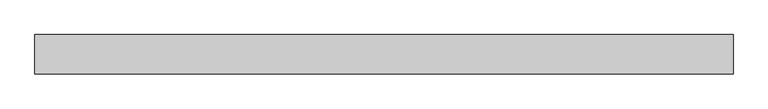
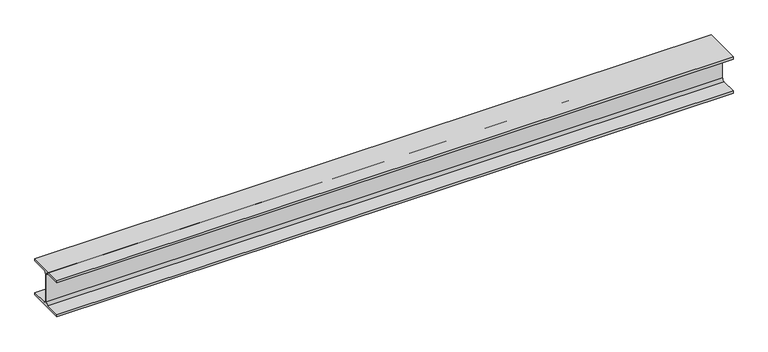
"""IFC4 building model written with IfcOpenShell, lengths in millimetres: beam geometry, 0912_Steel Framing_H-KSD3502 : H_SB_ASB_H-200x200x8x12."""

from ifc_helpers import new_model, si_unit, point, frame, frame_2d, origin, place, context, project, spatial, polyline, circle_curve, trimmed, segment, composite_curve, outline, extrude, source, transform, mapped, element, save


def beam_e80e70f2(model_context):
    return source(origin(), model_context, "Body", "SweptSolid", [
        extrude(outline(composite_curve([segment(polyline([(100.0, -88.0), (100.0, -100.0), (-100.0, -100.0), (-100.0, -88.0), (-17.0, -88.0)]), True, "CONTINUOUS"), segment(trimmed(circle_curve(frame_2d((-17.0, -75.0)), 13.0), [point((-17.0, -88.0))], [point((-4.0, -75.0))], True, "CARTESIAN"), True, "CONTINUOUS"), segment(polyline([(-4.0, -75.0), (-4.0, 75.0)]), True, "CONTINUOUS"), segment(trimmed(circle_curve(frame_2d((-17.0, 75.0)), 13.0), [point((-4.0, 75.0))], [point((-17.0, 88.0))], True, "CARTESIAN"), True, "CONTINUOUS"), segment(polyline([(-17.0, 88.0), (-100.0, 88.0), (-100.0, 100.0), (100.0, 100.0), (100.0, 88.0), (17.0, 88.0)]), True, "CONTINUOUS"), segment(trimmed(circle_curve(frame_2d((17.0, 75.0)), 13.0), [point((17.0, 88.0))], [point((4.0, 75.0))], True, "CARTESIAN"), True, "CONTINUOUS"), segment(polyline([(4.0, 75.0), (4.0, -75.0)]), True, "CONTINUOUS"), segment(trimmed(circle_curve(frame_2d((17.0, -75.0)), 13.0), [point((4.0, -75.0))], [point((17.0, -88.0))], True, "CARTESIAN"), True, "CONTINUOUS"), segment(polyline([(17.0, -88.0), (100.0, -88.0)]), True, "CONTINUOUS")], self_intersect=False)), frame((-1725.502423, 0.0, 0.0), z_axis=(1.0, 0.0, 0.0), x_axis=(0.0, 1.0, 0.0)), (0.0, 0.0, 1.0), 3536.3433078),
    ])


if __name__ == "__main__":
    model = new_model("IFC4")
    model_context = context("Model", 3, world=origin())
    ifc_project = project(units=[si_unit("LENGTHUNIT", "METRE", prefix="MILLI")], contexts=[model_context])
    site = spatial("IfcSite", under=ifc_project)
    building = spatial("IfcBuilding", under=site)
    placement = place(None, origin())
    beam_shape = beam_e80e70f2(model_context)
    element("IfcBeam", 1, ObjectType="0912_Steel Framing_H-KSD3502 : H_SB_ASB_H-200x200x8x12", at=placement, inside=building, context=model_context, shape_type="MappedRepresentation", body=[
        mapped(beam_shape, transform((0.0, 0.0, 0.0), x_axis=(1.0, 0.0, 0.0), y_axis=(0.0, 1.0, 0.0), z_axis=(0.0, 0.0, 1.0))),
    ])
    save(model, "model.ifc")

# Revit data of these elements
# Type "0912_Steel Framing_H-KSD3502 : H_SB_ASB_H-200x200x8x12"
#   H_WM Code_1 = "S01AA002-00001 | Main Steel Structure Fabrication Work | Shelter/Building | Medium Steel - Standard (90KG/M>Weight≥30KG/M) | Material: (   )"
#   H_WM Code_2 = "S03AA028-00001 | Main Steel Structure Erection Work | Shelter/Building | Medium Steel (90KG/M>Weight≥30KG/M) | Material: (   )"
#   H_WM Code_3 = "S01AA010-00001 | Main Steel Structure Fabrication Work | Shelter/Building | Steel Painting/Coating | for Non-Fireproofed Steel Surface, Surface Preparation, Primer, Second & Final Coat | Material: (   )"
#   H_Q'ty Cal Type Tag = "SB-Q2"
#   Width = 20.0 cm
#   Web Thickness = 0.8 cm
#   Web Fillet = 1.3 cm
#   Warping Constant = 141000.0 cm⁶
#   W = 0
#   Torsional Moment of Inertia = 26.2485 cm⁴
#   Section Area = 63.53 cm²
#   Plastic Modulus weak axis = 244.0 cm³
#   Plastic Modulus strong axis = 525.0 cm³
#   Perimeter = 1.16 m²/m
#   Nominal Weight = 49.90 kgf/m
#   Moment of Inertia weak axis = 1600.00 cm⁴
#   Moment of Inertia strong axis = 4720.00 cm⁴
#   Height = 20.0 cm
#   Flange Thickness = 1.2 cm
#   Elastic Modulus weak axis = 160.0 cm³
#   Elastic Modulus strong axis = 472.0 cm³
#   Centroid Vertical = 10.0 cm
#   Centroid Horizontal = 10.0 cm
#   Ix = 47200000
#   Length [instance default] = 1.5240 m
#   Zx = 525000
#   b = 0.2000 m
#   h = 0.2000 m
#   r = 0.0130 m
#   s = 0.0080 m
#   t = 0.0120 m
#   A = 0.006353 m²
#   Structural Material [instance default] = Steel, 45-345
#   Assembly Code = ""
# Element 1 (IfcBeam, "0912_Steel Framing_H-KSD3502 : H_SB_ASB_H-200x200x8x12")
#   Structural Material = none
# Materials
#   "Steel, 45-345": class "Metal", colour RGB 189 187 185, transparency 0, Description = "Steel 345 MPa", Cost = 0
